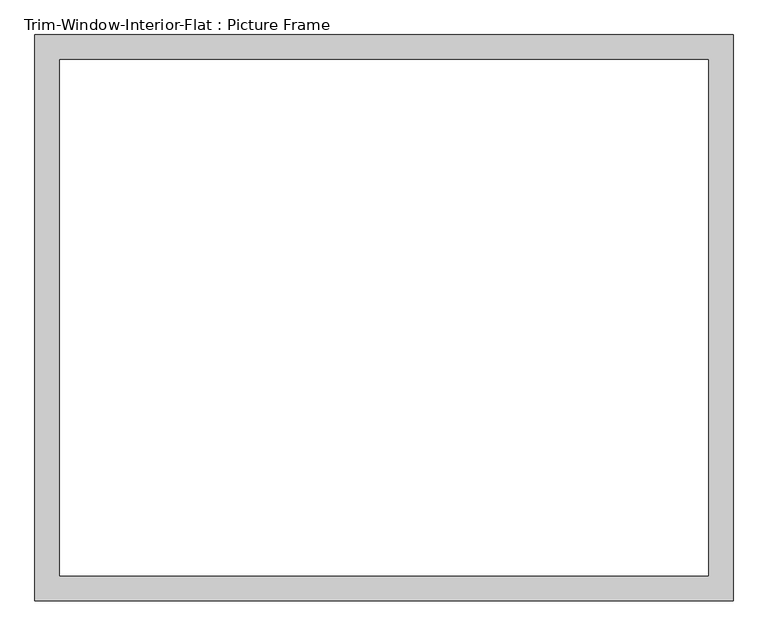
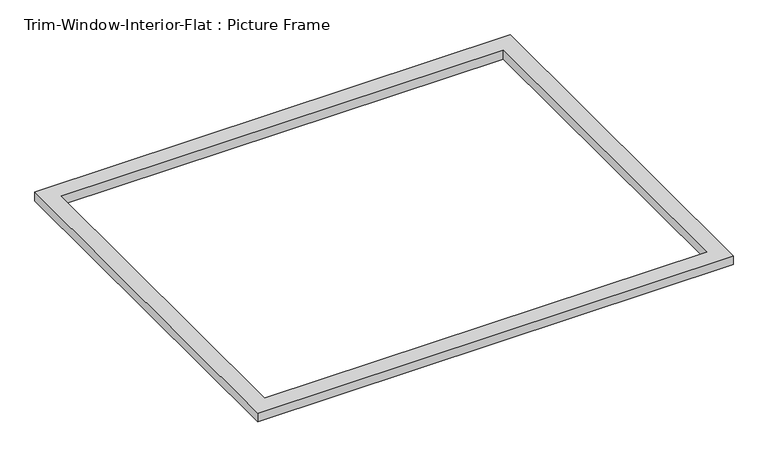
"""IFC4 building model written with IfcOpenShell, lengths in millimetres: proxy geometry, Trim-Window-Interior-Flat : Picture Frame."""

import ifcopenshell
import ifcopenshell.guid

model = None  # the IFC model being written
_history = None  # IfcOwnerHistory: only IFC2X3 demands one
_inside = {}  # id of a spatial element -> (the spatial element, [elements in it])
_under = {}  # id of a project, library or spatial element -> (it, [spatial elements below it])
_declared = {}  # id of a project -> (the project, [libraries it declares])
_typed = {}  # id of a type object -> (the type object, [elements of that type])
_made_of = {}  # id of a material, layer set ... -> (it, [elements and type objects made of it])


def new_model(schema):
    """Start an empty IFC model of exactly this schema.

    Asked for "IFC4X3", IfcOpenShell would pick the latest addendum, in which some entities
    have other attributes; the version numbers below select the first issue.
    IFC2X3 requires an IfcOwnerHistory on every rooted entity: one is made here for all.
    """
    global model, _history
    if schema == "IFC4X3":
        model = ifcopenshell.file(schema_version=(4, 3, 0, 0))
    else:
        model = ifcopenshell.file(schema=schema)
    _inside.clear()
    _under.clear()
    _declared.clear()
    _typed.clear()
    _made_of.clear()
    _history = None
    if model.schema == "IFC2X3":
        org = make("IfcOrganization", Name="unknown")
        user = make(
            "IfcPersonAndOrganization",
            ThePerson=make("IfcPerson", FamilyName="unknown"),
            TheOrganization=org,
        )
        app = make(
            "IfcApplication",
            ApplicationDeveloper=org,
            Version="unknown",
            ApplicationFullName="unknown",
            ApplicationIdentifier="unknown",
        )
        _history = make(
            "IfcOwnerHistory",
            OwningUser=user,
            OwningApplication=app,
            ChangeAction="ADDED",
            CreationDate=0,
        )
    return model


def make(cls, **values):
    """One entity of the class cls with the attributes given. An attribute that is None is left unset."""
    return model.create_entity(
        cls, **{name: value for name, value in values.items() if value is not None}
    )


def rooted(cls, **values):
    """An entity with a GlobalId (a new one), such as an element, a storey or a relation."""
    return make(cls, GlobalId=ifcopenshell.guid.new(), OwnerHistory=_history, **values)


def si_unit(unit_type, name, prefix=None):
    """IfcSIUnit, for example si_unit("LENGTHUNIT", "METRE", prefix="MILLI")."""
    return make("IfcSIUnit", UnitType=unit_type, Prefix=prefix, Name=name)


def assignment(units):
    """IfcUnitAssignment: the units of a project."""
    return None if units is None else make("IfcUnitAssignment", Units=units)


def point(xyz):
    """IfcCartesianPoint."""
    return None if xyz is None else make("IfcCartesianPoint", Coordinates=xyz)


def direction(xyz):
    """IfcDirection."""
    return None if xyz is None else make("IfcDirection", DirectionRatios=xyz)


def frame(location, z_axis=None, x_axis=None):
    """IfcAxis2Placement3D, a coordinate frame: its origin and axes. An axis left out is left unset."""
    return make(
        "IfcAxis2Placement3D",
        Location=point(location),
        Axis=direction(z_axis),
        RefDirection=direction(x_axis),
    )


def origin():
    """The frame at (0, 0, 0) with its axes left unset."""
    return frame((0.0, 0.0, 0.0))


def origin_with_axes():
    """The frame at (0, 0, 0) with the z axis (0, 0, 1) and the x axis (1, 0, 0) written out."""
    return frame((0.0, 0.0, 0.0), z_axis=(0.0, 0.0, 1.0), x_axis=(1.0, 0.0, 0.0))


def place(relative_to, where):
    """IfcLocalPlacement: puts the frame where relative to a parent placement (None: the world)."""
    return make(
        "IfcLocalPlacement", PlacementRelTo=relative_to, RelativePlacement=where
    )


def context(
    kind, dimensions, precision=None, world=None, true_north=None, identifier=None
):
    """IfcGeometricRepresentationContext, for example the 3D "Model" context."""
    return make(
        "IfcGeometricRepresentationContext",
        ContextIdentifier=identifier,
        ContextType=kind,
        CoordinateSpaceDimension=dimensions,
        Precision=precision,
        WorldCoordinateSystem=world,
        TrueNorth=true_north,
    )


def project(units=None, contexts=None):
    """IfcProject with its units and contexts."""
    return rooted(
        "IfcProject",
        Name="project",
        RepresentationContexts=contexts,
        UnitsInContext=assignment(units),
    )


def spatial(cls, under=None, at=None, **own):
    """A site, building, storey or space (cls), placed at a placement, below another one or the project."""
    s = rooted(cls, ObjectPlacement=at, **own)
    if under is not None:
        _under.setdefault(under.id(), (under, []))[1].append(s)
    return s


def polyline(points):
    """IfcPolyline through the points."""
    return make("IfcPolyline", Points=[point(p) for p in points])


def outline(outer, holes=None, kind="AREA"):
    """IfcArbitraryClosedProfileDef: a profile drawn as a closed curve; with holes, ...WithVoids."""
    if holes is None:
        return make("IfcArbitraryClosedProfileDef", ProfileType=kind, OuterCurve=outer)
    return make(
        "IfcArbitraryProfileDefWithVoids",
        ProfileType=kind,
        OuterCurve=outer,
        InnerCurves=holes,
    )


def extrude(swept, where, along, depth):
    """IfcExtrudedAreaSolid: the profile swept, set in the frame where, extruded along a direction by depth."""
    return make(
        "IfcExtrudedAreaSolid",
        SweptArea=swept,
        Position=where,
        ExtrudedDirection=direction(along),
        Depth=depth,
    )


def shape(context_of_items, identifier, shape_type, items):
    """IfcShapeRepresentation: the items that make up one representation, for example the "Body"."""
    return make(
        "IfcShapeRepresentation",
        ContextOfItems=context_of_items,
        RepresentationIdentifier=identifier,
        RepresentationType=shape_type,
        Items=items,
    )


def source(mapping_origin, context_of_items, identifier, shape_type, items):
    """IfcRepresentationMap: a shape defined once, which mapped items show again and again."""
    return make(
        "IfcRepresentationMap",
        MappingOrigin=mapping_origin,
        MappedRepresentation=shape(context_of_items, identifier, shape_type, items),
    )


def transform(
    local_origin,
    x_axis=None,
    y_axis=None,
    z_axis=None,
    scale=None,
    scale2=None,
    scale3=None,
    uniform=True,
):
    """IfcCartesianTransformationOperator3D, or its non-uniform kind. x_axis, y_axis, z_axis: its Axis1, 2, 3."""
    if uniform:
        return make(
            "IfcCartesianTransformationOperator3D",
            Axis1=direction(x_axis),
            Axis2=direction(y_axis),
            LocalOrigin=point(local_origin),
            Scale=scale,
            Axis3=direction(z_axis),
        )
    return make(
        "IfcCartesianTransformationOperator3DnonUniform",
        Axis1=direction(x_axis),
        Axis2=direction(y_axis),
        LocalOrigin=point(local_origin),
        Scale=scale,
        Axis3=direction(z_axis),
        Scale2=scale2,
        Scale3=scale3,
    )


def mapped(mapping_source, mapping_target):
    """IfcMappedItem: shows the shape of a source again, moved by a transform."""
    return make(
        "IfcMappedItem", MappingSource=mapping_source, MappingTarget=mapping_target
    )


def made_of(thing, what):
    """Note that an element or type object is made of a material, layer set ...; save() writes the relation."""
    if what is not None:
        _made_of.setdefault(what.id(), (what, []))[1].append(thing)
    return thing


def element(
    cls,
    number,
    at=None,
    inside=None,
    cuts=None,
    type_object=None,
    material=None,
    context=None,
    identifier="Body",
    shape_type=None,
    held_by="IfcProductDefinitionShape",
    body=None,
    shapes=None,
    **own,
):
    """One element of the class cls, such as IfcWall. Its Tag is "e" and its number.

    at: its placement. inside: the storey or other place that contains it. cuts: it is an
    opening in that element (IfcRelVoidsElement). A single representation is given by context,
    identifier, shape_type and body (its items); several are given by shapes. held_by: the class
    of the entity that holds the representations. save() writes the other relations.
    """
    e = rooted(cls, Tag="e%d" % number, ObjectPlacement=at, **own)
    if body is not None:
        shapes = [shape(context, identifier, shape_type, body)]
    if shapes is not None:
        e.Representation = make(held_by, Representations=shapes)
    if inside is not None:
        _inside.setdefault(inside.id(), (inside, []))[1].append(e)
    if cuts is not None:
        rooted(
            "IfcRelVoidsElement", RelatingBuildingElement=cuts, RelatedOpeningElement=e
        )
    if type_object is not None:
        _typed.setdefault(type_object.id(), (type_object, []))[1].append(e)
    return made_of(e, material)


def aggregate(whole, parts):
    """IfcRelAggregates: a whole, such as a stair, and the parts it consists of."""
    return rooted("IfcRelAggregates", RelatingObject=whole, RelatedObjects=parts)


def save(model, path):
    """Write the relations noted so far, then the file.

    IfcRelAggregates (storeys below a building ...), IfcRelContainedInSpatialStructure (elements
    in a storey), IfcRelDefinesByType, IfcRelAssociatesMaterial and IfcRelDeclares: one each for
    every whole, place, type object, material and project.
    """
    for whole, parts in _under.values():
        aggregate(whole, parts)
    for where, things in _inside.values():
        rooted(
            "IfcRelContainedInSpatialStructure",
            RelatedElements=things,
            RelatingStructure=where,
        )
    for kind, things in _typed.values():
        rooted("IfcRelDefinesByType", RelatedObjects=things, RelatingType=kind)
    for what, things in _made_of.values():
        rooted("IfcRelAssociatesMaterial", RelatedObjects=things, RelatingMaterial=what)
    for by, libraries in _declared.values():
        rooted("IfcRelDeclares", RelatingContext=by, RelatedDefinitions=libraries)
    model.write(path)


def trim_window_interior_flat_picture_frame_0f2e31f9(model_context):
    return source(origin(), model_context, "Body", "SweptSolid", [
        extrude(outline(polyline([(806.45, 44.45), (806.45, -1263.65), (-806.45, -1263.65), (-806.45, 44.45), (806.45, 44.45)]), holes=[polyline([(749.3, -12.7), (-749.3, -12.7), (-749.3, -1206.5), (749.3, -1206.5), (749.3, -12.7)])]), origin_with_axes(), (0.0, 0.0, 1.0), 31.75),
    ])


if __name__ == "__main__":
    model = new_model("IFC4")
    model_context = context("Model", 3, world=origin())
    ifc_project = project(units=[si_unit("LENGTHUNIT", "METRE", prefix="MILLI")], contexts=[model_context])
    site = spatial("IfcSite", under=ifc_project)
    building = spatial("IfcBuilding", under=site)
    placement = place(None, origin())
    trim_window_interior_flat_picture_frame_shape = trim_window_interior_flat_picture_frame_0f2e31f9(model_context)
    element("IfcBuildingElementProxy", 1, Name="Trim-Window-Interior-Flat : Picture Frame", ObjectType="Trim-Window-Interior-Flat : Picture Frame", at=placement, inside=building, context=model_context, shape_type="MappedRepresentation", body=[
        mapped(trim_window_interior_flat_picture_frame_shape, transform((0.0, 0.0, 0.0), x_axis=(1.0, 0.0, 0.0), y_axis=(0.0, 1.0, 0.0), z_axis=(0.0, 0.0, 1.0))),
    ])
    save(model, "model.ifc")

# Revit data of these elements
# Type "Trim-Window-Interior-Flat : Picture Frame"
#   Trim Thickness_Picture Frame = 0' - 1 1/4"
#   Trim Width = 0' - 2 1/4"
#   Trim Thickness_with Sill = 0' - 0 3/4"
#   Sill Thickness = 0' - 1 1/4"
#   Opening Width [instance default] = 2' - 0"
#   Opening Height [instance default] = 3' - 0"
#   Default Elevation = 4' - 0"
#   Sill = no
#   Picture Frame = yes
#   Trim Material [instance default] = none
# Element 1 (IfcBuildingElementProxy, "Trim-Window-Interior-Flat : Picture Frame")
#   Opening Width = 5' - 0"
#   Opening Height = 4' - 0"
#   Trim Material = Cherry
#   Materials on its faces: "Cherry"
# Materials
#   "Cherry": class "Wood", colour RGB 157 77 38, transparency 0, Description = "Prunus Serotina", Cost = 0
